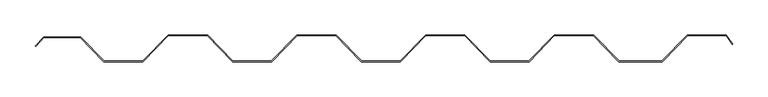
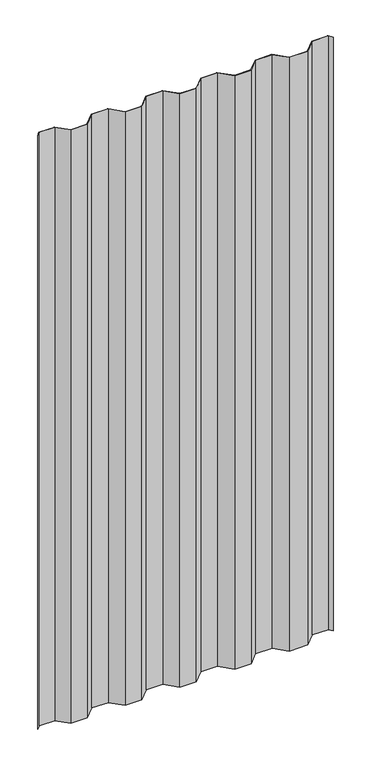
"""IFC4 building model written with IfcOpenShell, lengths in millimetres: proxy geometry, Generic Models 2:Generic Models 2:310765:Generic Models 2:310765 : Generic Models 2:Generic Models 2:310765:282 : Generic Models 2:Generic Models 2:310765:Generic Models 2:310765 : Generic Models 2:Generic Models 2:310765:300385."""

from ifc_helpers import new_model, si_unit, frame, origin, place, context, project, spatial, polyline, outline, extrude, source, transform, mapped, element, save


def generic_models_223ea8f1(model_context):
    return source(origin(), model_context, "Body", "SweptSolid", [
        extrude(outline(polyline([(793296.6908851, -578743.0895469), (793349.2846908, -578743.0895469), (793382.9166755, -578777.6476341), (793437.4250755, -578777.6476341), (793473.5872672, -578740.3413841), (793529.6344839, -578740.3413841), (793565.7966755, -578777.6476341), (793620.3050755, -578777.6476341), (793656.4672672, -578740.3413841), (793712.5144839, -578740.3413841), (793748.6766755, -578777.6476341), (793803.1850755, -578777.6476341), (793839.3472672, -578740.3413841), (793895.3944839, -578740.3413841), (793931.5566755, -578777.6476341), (793986.0650755, -578777.6476341), (794022.2272672, -578740.3413841), (794078.2744839, -578740.3413841), (794114.4366755, -578777.6476341), (794175.2950755, -578777.6476341), (794211.4572672, -578740.3413841), (794266.7350755, -578740.3413841), (794275.9134457, -578753.4494551), (794275.2632437, -578753.9047314), (794266.3218754, -578741.1351341), (794211.7933127, -578741.1351341), (794175.6311211, -578778.4413841), (794114.10063, -578778.4413841), (794077.9384383, -578741.1351341), (794022.5633127, -578741.1351341), (793986.4011211, -578778.4413841), (793931.22063, -578778.4413841), (793895.0584383, -578741.1351341), (793839.6833127, -578741.1351341), (793803.5211211, -578778.4413841), (793748.34063, -578778.4413841), (793712.1784383, -578741.1351341), (793656.8033127, -578741.1351341), (793620.6411211, -578778.4413841), (793565.46063, -578778.4413841), (793529.2984383, -578741.1351341), (793473.9233127, -578741.1351341), (793437.7611211, -578778.4413841), (793382.5815612, -578778.4413841), (793348.9495764, -578743.8832969), (793297.0432224, -578743.8832969), (793285.3971106, -578756.7595897), (793284.8351388, -578756.1976179), (793296.6908851, -578743.0895469)])), frame((0.0, 0.0, 4033.8810286), z_axis=(0.0, 0.0, 1.0), x_axis=(1.0, 0.0, 0.0)), (0.0, 0.0, 1.0), 2100.2189714),
    ])


if __name__ == "__main__":
    model = new_model("IFC4")
    model_context = context("Model", 3, world=origin())
    ifc_project = project(units=[si_unit("LENGTHUNIT", "METRE", prefix="MILLI")], contexts=[model_context])
    site = spatial("IfcSite", under=ifc_project)
    building = spatial("IfcBuilding", under=site)
    placement = place(None, origin())
    generic_models_shape = generic_models_223ea8f1(model_context)
    element("IfcBuildingElementProxy", 1, Name="Generic Models 2:Generic Models 2:310765:Generic Models 2:310765 : Generic Models 2:Generic Models 2:310765:282 : Generic Models 2:Generic Models 2:310765:Generic Models 2:310765 : Generic Models 2:Generic Models 2:310765:300385", ObjectType="Generic Models 2:Generic Models 2:310765:Generic Models 2:310765 : Generic Models 2:Generic Models 2:310765:282 : Generic Models 2:Generic Models 2:310765:Generic Models 2:310765 : Generic Models 2:Generic Models 2:310765:300385", at=placement, inside=building, context=model_context, shape_type="MappedRepresentation", body=[
        mapped(generic_models_shape, transform((0.0, 0.0, 0.0), x_axis=(1.0, 0.0, 0.0), y_axis=(0.0, 1.0, 0.0), z_axis=(0.0, 0.0, 1.0))),
    ])
    save(model, "model.ifc")

# Revit data of these elements
# Type "Generic Models 2:Generic Models 2:310765:Generic Models 2:310765 : Generic Models 2:Generic Models 2:310765:282 : Generic Models 2:Generic Models 2:310765:Generic Models 2:310765 : Generic Models 2:Generic Models 2:310765:300385"
#   NameOverride = "Generic Models 2:Generic Models 2:310765:Generic Models 2:310765 : Generic Models 2:Generic Models 2:310765:300385"
#   ObjectTypeOverride = "Generic Models 2:310765 : Generic Models 2:Generic Models 2:310765"
#   Reference = "Generic Models 2"
#   Tag = "300385"
# Element 1 (IfcBuildingElementProxy, "Generic Models 2:Generic Models 2:310765:Generic Models 2:310765 : Generic Models 2:Generic Models 2:310765:282 : Generic Models 2:Generic Models 2:310765:Generic Models 2:310765 : Generic Models 2:Generic Models 2:310765:300385")
#   Materials on its faces: "VERTICAL CORRUGATED METAL PANEL - EXPOSED FASTENERS - (MBCI 7.2 PANEL)"
# Materials
#   "VERTICAL CORRUGATED METAL PANEL - EXPOSED FASTENERS - (MBCI 7.2 PANEL)": class "Generic", colour RGB 120 120 120, transparency 0, Cost = 0
